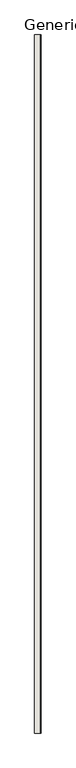
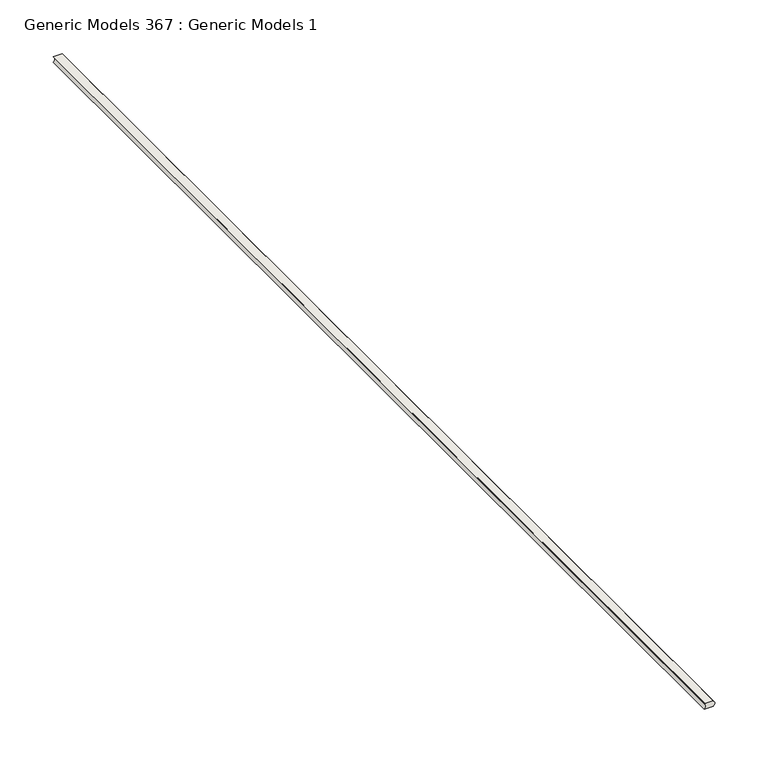
"""IFC4 building model written with IfcOpenShell, lengths in millimetres: wall geometry, Generic Models 367 : Generic Models 1."""

from ifc_helpers import new_model, si_unit, point, frame, frame_2d, origin, place, context, project, spatial, polyline, circle_curve, trimmed, segment, composite_curve, outline, extrude, source, transform, mapped, element, save


def generic_models_367_generic_models_1_45e5e002(model_context):
    return source(origin(), model_context, "Body", "SweptSolid", [
        extrude(outline(composite_curve([segment(trimmed(circle_curve(frame_2d((2454.275, 137458.7102595)), 4.3100275), [point((2457.45, 137461.625))], [point((2451.1, 137461.625))], True, "CARTESIAN"), True, "CONTINUOUS"), segment(polyline([(2451.1, 137461.625), (2451.1, 137471.15)]), True, "CONTINUOUS"), segment(trimmed(circle_curve(frame_2d((2454.275, 137468.2352595)), 4.3100275), [point((2451.1, 137471.15))], [point((2457.45, 137471.15))], False, "CARTESIAN"), True, "CONTINUOUS"), segment(polyline([(2457.45, 137471.15), (2457.45, 137461.625)]), True, "CONTINUOUS")], self_intersect=False)), frame((0.0, 0.0, 0.0), z_axis=(0.0, 1.0, 0.0), x_axis=(0.0, 0.0, 1.0)), (0.0, 0.0, 1.0), 1219.2),
    ])


if __name__ == "__main__":
    model = new_model("IFC4")
    model_context = context("Model", 3, world=origin())
    ifc_project = project(units=[si_unit("LENGTHUNIT", "METRE", prefix="MILLI")], contexts=[model_context])
    site = spatial("IfcSite", under=ifc_project)
    building = spatial("IfcBuilding", under=site)
    placement = place(None, origin())
    generic_models_367_generic_models_1_shape = generic_models_367_generic_models_1_45e5e002(model_context)
    element("IfcWall", 1, ObjectType="Generic Models 367 : Generic Models 1", at=placement, inside=building, context=model_context, shape_type="MappedRepresentation", body=[
        mapped(generic_models_367_generic_models_1_shape, transform((0.0, 0.0, 0.0), x_axis=(1.0, 0.0, 0.0), y_axis=(0.0, 1.0, 0.0), z_axis=(0.0, 0.0, 1.0))),
    ])
    save(model, "model.ifc")

# Revit data of these elements
# Element 1 (IfcWall, "Generic Models 367 : Generic Models 1")
#   Materials on its faces: "CONTINUOUS FIRE RATED SEALANT EACH SIDE."
# Materials
#   "CONTINUOUS FIRE RATED SEALANT EACH SIDE.": class "Miscellaneous", colour RGB 127 127 127, transparency 0, Cost = 0
